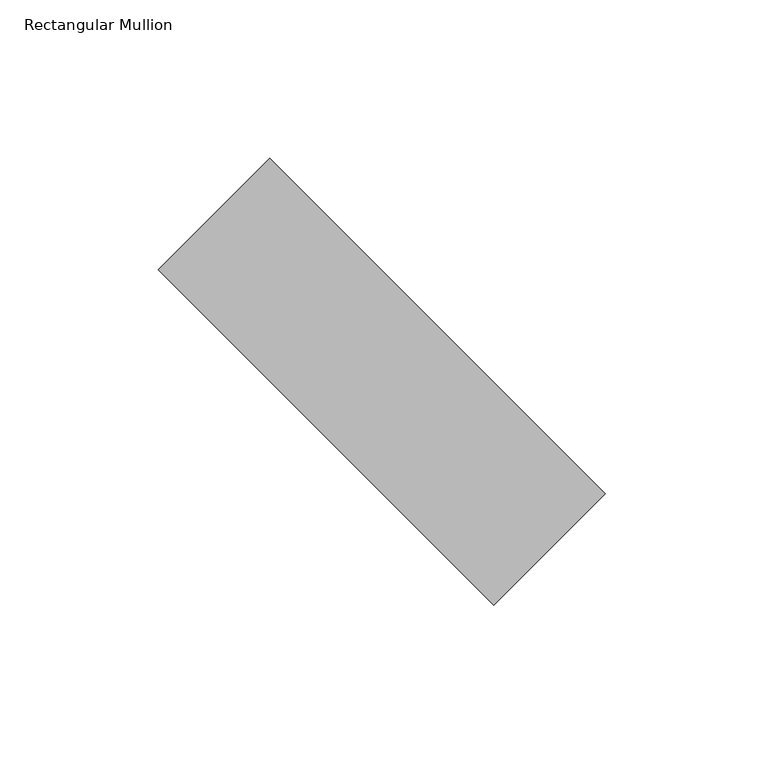
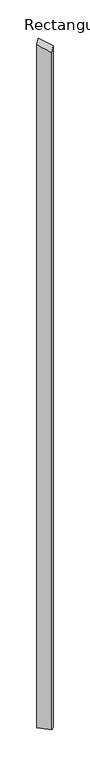
"""IFC4 building model written with IfcOpenShell, lengths in millimetres: member geometry, Rectangular Mullion : tilted mullions."""

import ifcopenshell
import ifcopenshell.guid

model = None  # the IFC model being written
_history = None  # IfcOwnerHistory: only IFC2X3 demands one
_inside = {}  # id of a spatial element -> (the spatial element, [elements in it])
_under = {}  # id of a project, library or spatial element -> (it, [spatial elements below it])
_declared = {}  # id of a project -> (the project, [libraries it declares])
_typed = {}  # id of a type object -> (the type object, [elements of that type])
_made_of = {}  # id of a material, layer set ... -> (it, [elements and type objects made of it])


def new_model(schema):
    """Start an empty IFC model of exactly this schema.

    Asked for "IFC4X3", IfcOpenShell would pick the latest addendum, in which some entities
    have other attributes; the version numbers below select the first issue.
    IFC2X3 requires an IfcOwnerHistory on every rooted entity: one is made here for all.
    """
    global model, _history
    if schema == "IFC4X3":
        model = ifcopenshell.file(schema_version=(4, 3, 0, 0))
    else:
        model = ifcopenshell.file(schema=schema)
    _inside.clear()
    _under.clear()
    _declared.clear()
    _typed.clear()
    _made_of.clear()
    _history = None
    if model.schema == "IFC2X3":
        org = make("IfcOrganization", Name="unknown")
        user = make(
            "IfcPersonAndOrganization",
            ThePerson=make("IfcPerson", FamilyName="unknown"),
            TheOrganization=org,
        )
        app = make(
            "IfcApplication",
            ApplicationDeveloper=org,
            Version="unknown",
            ApplicationFullName="unknown",
            ApplicationIdentifier="unknown",
        )
        _history = make(
            "IfcOwnerHistory",
            OwningUser=user,
            OwningApplication=app,
            ChangeAction="ADDED",
            CreationDate=0,
        )
    return model


def make(cls, **values):
    """One entity of the class cls with the attributes given. An attribute that is None is left unset."""
    return model.create_entity(
        cls, **{name: value for name, value in values.items() if value is not None}
    )


def rooted(cls, **values):
    """An entity with a GlobalId (a new one), such as an element, a storey or a relation."""
    return make(cls, GlobalId=ifcopenshell.guid.new(), OwnerHistory=_history, **values)


def si_unit(unit_type, name, prefix=None):
    """IfcSIUnit, for example si_unit("LENGTHUNIT", "METRE", prefix="MILLI")."""
    return make("IfcSIUnit", UnitType=unit_type, Prefix=prefix, Name=name)


def assignment(units):
    """IfcUnitAssignment: the units of a project."""
    return None if units is None else make("IfcUnitAssignment", Units=units)


def point(xyz):
    """IfcCartesianPoint."""
    return None if xyz is None else make("IfcCartesianPoint", Coordinates=xyz)


def direction(xyz):
    """IfcDirection."""
    return None if xyz is None else make("IfcDirection", DirectionRatios=xyz)


def frame(location, z_axis=None, x_axis=None):
    """IfcAxis2Placement3D, a coordinate frame: its origin and axes. An axis left out is left unset."""
    return make(
        "IfcAxis2Placement3D",
        Location=point(location),
        Axis=direction(z_axis),
        RefDirection=direction(x_axis),
    )


def origin():
    """The frame at (0, 0, 0) with its axes left unset."""
    return frame((0.0, 0.0, 0.0))


def place(relative_to, where):
    """IfcLocalPlacement: puts the frame where relative to a parent placement (None: the world)."""
    return make(
        "IfcLocalPlacement", PlacementRelTo=relative_to, RelativePlacement=where
    )


def context(
    kind, dimensions, precision=None, world=None, true_north=None, identifier=None
):
    """IfcGeometricRepresentationContext, for example the 3D "Model" context."""
    return make(
        "IfcGeometricRepresentationContext",
        ContextIdentifier=identifier,
        ContextType=kind,
        CoordinateSpaceDimension=dimensions,
        Precision=precision,
        WorldCoordinateSystem=world,
        TrueNorth=true_north,
    )


def project(units=None, contexts=None):
    """IfcProject with its units and contexts."""
    return rooted(
        "IfcProject",
        Name="project",
        RepresentationContexts=contexts,
        UnitsInContext=assignment(units),
    )


def spatial(cls, under=None, at=None, **own):
    """A site, building, storey or space (cls), placed at a placement, below another one or the project."""
    s = rooted(cls, ObjectPlacement=at, **own)
    if under is not None:
        _under.setdefault(under.id(), (under, []))[1].append(s)
    return s


def faces_of(points, faces, orient=None, outer=None):
    """IfcFace entities. A face is a list of loops; a loop is a list of indices into points, from 0.

    orient and outer hold one flag for each loop. By default every Orientation is true, the
    first loop of a face is its IfcFaceOuterBound and the others are IfcFaceBound.
    """
    made = []
    for i, loops in enumerate(faces):
        bounds = []
        for j, loop in enumerate(loops):
            is_outer = j == 0 if outer is None else outer[i][j]
            bounds.append(
                make(
                    "IfcFaceOuterBound" if is_outer else "IfcFaceBound",
                    Bound=make("IfcPolyLoop", Polygon=[points[k] for k in loop]),
                    Orientation=True if orient is None else orient[i][j],
                )
            )
        made.append(make("IfcFace", Bounds=bounds))
    return made


def faceted_brep(points, faces, orient=None, outer=None, voids=None):
    """IfcFacetedBrep: a solid bounded by flat faces; with voids (closed shells), ...WithVoids."""
    shared = [point(p) for p in points]
    hull = make("IfcClosedShell", CfsFaces=faces_of(shared, faces, orient, outer))
    if voids is None:
        return make("IfcFacetedBrep", Outer=hull)
    return make(
        "IfcFacetedBrepWithVoids",
        Outer=hull,
        Voids=[
            make(cls, CfsFaces=faces_of(shared, fs, o, b)) for cls, fs, o, b in voids
        ],
    )


def shape(context_of_items, identifier, shape_type, items):
    """IfcShapeRepresentation: the items that make up one representation, for example the "Body"."""
    return make(
        "IfcShapeRepresentation",
        ContextOfItems=context_of_items,
        RepresentationIdentifier=identifier,
        RepresentationType=shape_type,
        Items=items,
    )


def source(mapping_origin, context_of_items, identifier, shape_type, items):
    """IfcRepresentationMap: a shape defined once, which mapped items show again and again."""
    return make(
        "IfcRepresentationMap",
        MappingOrigin=mapping_origin,
        MappedRepresentation=shape(context_of_items, identifier, shape_type, items),
    )


def transform(
    local_origin,
    x_axis=None,
    y_axis=None,
    z_axis=None,
    scale=None,
    scale2=None,
    scale3=None,
    uniform=True,
):
    """IfcCartesianTransformationOperator3D, or its non-uniform kind. x_axis, y_axis, z_axis: its Axis1, 2, 3."""
    if uniform:
        return make(
            "IfcCartesianTransformationOperator3D",
            Axis1=direction(x_axis),
            Axis2=direction(y_axis),
            LocalOrigin=point(local_origin),
            Scale=scale,
            Axis3=direction(z_axis),
        )
    return make(
        "IfcCartesianTransformationOperator3DnonUniform",
        Axis1=direction(x_axis),
        Axis2=direction(y_axis),
        LocalOrigin=point(local_origin),
        Scale=scale,
        Axis3=direction(z_axis),
        Scale2=scale2,
        Scale3=scale3,
    )


def mapped(mapping_source, mapping_target):
    """IfcMappedItem: shows the shape of a source again, moved by a transform."""
    return make(
        "IfcMappedItem", MappingSource=mapping_source, MappingTarget=mapping_target
    )


def made_of(thing, what):
    """Note that an element or type object is made of a material, layer set ...; save() writes the relation."""
    if what is not None:
        _made_of.setdefault(what.id(), (what, []))[1].append(thing)
    return thing


def element(
    cls,
    number,
    at=None,
    inside=None,
    cuts=None,
    type_object=None,
    material=None,
    context=None,
    identifier="Body",
    shape_type=None,
    held_by="IfcProductDefinitionShape",
    body=None,
    shapes=None,
    **own,
):
    """One element of the class cls, such as IfcWall. Its Tag is "e" and its number.

    at: its placement. inside: the storey or other place that contains it. cuts: it is an
    opening in that element (IfcRelVoidsElement). A single representation is given by context,
    identifier, shape_type and body (its items); several are given by shapes. held_by: the class
    of the entity that holds the representations. save() writes the other relations.
    """
    e = rooted(cls, Tag="e%d" % number, ObjectPlacement=at, **own)
    if body is not None:
        shapes = [shape(context, identifier, shape_type, body)]
    if shapes is not None:
        e.Representation = make(held_by, Representations=shapes)
    if inside is not None:
        _inside.setdefault(inside.id(), (inside, []))[1].append(e)
    if cuts is not None:
        rooted(
            "IfcRelVoidsElement", RelatingBuildingElement=cuts, RelatedOpeningElement=e
        )
    if type_object is not None:
        _typed.setdefault(type_object.id(), (type_object, []))[1].append(e)
    return made_of(e, material)


def aggregate(whole, parts):
    """IfcRelAggregates: a whole, such as a stair, and the parts it consists of."""
    return rooted("IfcRelAggregates", RelatingObject=whole, RelatedObjects=parts)


def save(model, path):
    """Write the relations noted so far, then the file.

    IfcRelAggregates (storeys below a building ...), IfcRelContainedInSpatialStructure (elements
    in a storey), IfcRelDefinesByType, IfcRelAssociatesMaterial and IfcRelDeclares: one each for
    every whole, place, type object, material and project.
    """
    for whole, parts in _under.values():
        aggregate(whole, parts)
    for where, things in _inside.values():
        rooted(
            "IfcRelContainedInSpatialStructure",
            RelatedElements=things,
            RelatingStructure=where,
        )
    for kind, things in _typed.values():
        rooted("IfcRelDefinesByType", RelatedObjects=things, RelatingType=kind)
    for what, things in _made_of.values():
        rooted("IfcRelAssociatesMaterial", RelatedObjects=things, RelatingMaterial=what)
    for by, libraries in _declared.values():
        rooted("IfcRelDeclares", RelatingContext=by, RelatedDefinitions=libraries)
    model.write(path)


def rectangular_mullion_fa86b804(model_context):
    return source(origin(), model_context, "Body", "Brep", [
        faceted_brep([(-35.3553391, 70.7106781, -7999.7416202), (70.7106781, -35.3553391, -7999.7416202), (35.3553391, -70.7106781, -7999.7416202), (-70.7106781, 35.3553391, -7999.7416202), (-70.7106781, 35.3553391, 9.9810707), (-35.3553391, 70.7106781, 55.0394649), (35.3553391, -70.7106781, -55.0394649), (70.7106781, -35.3553391, -9.9810707)], [[[0, 1, 2, 3]], [[4, 5, 0, 3]], [[6, 4, 3, 2]], [[7, 6, 2, 1]], [[5, 7, 1, 0]], [[5, 4, 6, 7]]]),
    ])


if __name__ == "__main__":
    model = new_model("IFC4")
    model_context = context("Model", 3, world=origin())
    ifc_project = project(units=[si_unit("LENGTHUNIT", "METRE", prefix="MILLI")], contexts=[model_context])
    site = spatial("IfcSite", under=ifc_project)
    building = spatial("IfcBuilding", under=site)
    placement = place(None, origin())
    rectangular_mullion_shape = rectangular_mullion_fa86b804(model_context)
    element("IfcMember", 1, ObjectType="Rectangular Mullion : tilted mullions", at=placement, inside=building, context=model_context, shape_type="MappedRepresentation", body=[
        mapped(rectangular_mullion_shape, transform((0.0, 0.0, 0.0), x_axis=(1.0, 0.0, 0.0), y_axis=(0.0, 1.0, 0.0), z_axis=(0.0, 0.0, 1.0))),
    ])
    save(model, "model.ifc")

# Revit data of these elements
# Type "Rectangular Mullion : tilted mullions"
#   built-in parameter 1007304 = 0.492126 (stored number, unit not read)
#   built-in parameter 1007301 = 0.082021 (stored number, unit not read)
#   built-in parameter 1007300 = 0.082021 (stored number, unit not read)
# Element 1 (IfcMember, "Rectangular Mullion : tilted mullions")
#   Materials on its faces: "Aluminum"
# Materials
#   "Aluminum": class "Metal", colour RGB 244 244 244, transparency 0, Description = "Aluminum 6061", Cost = 0
